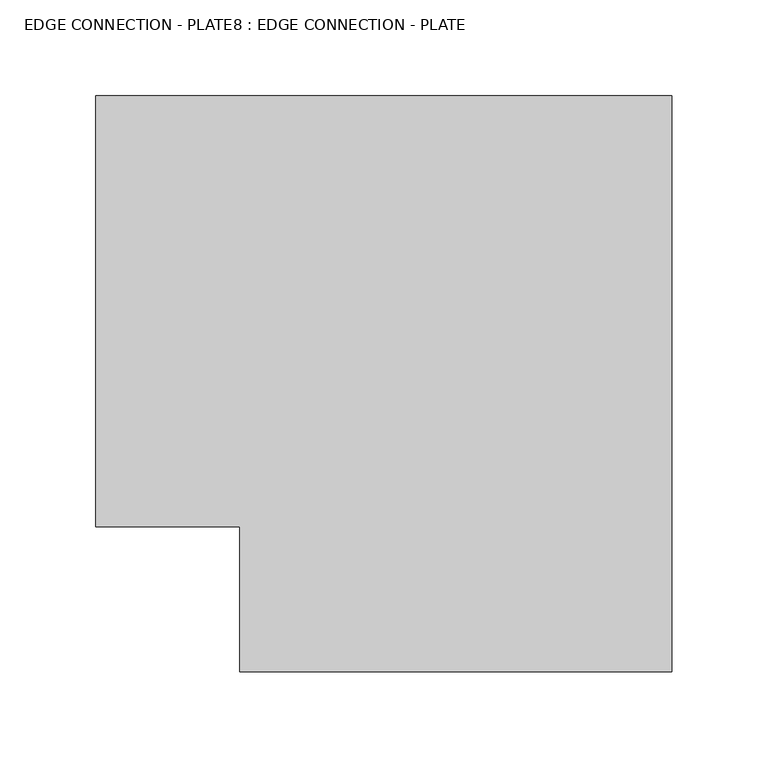
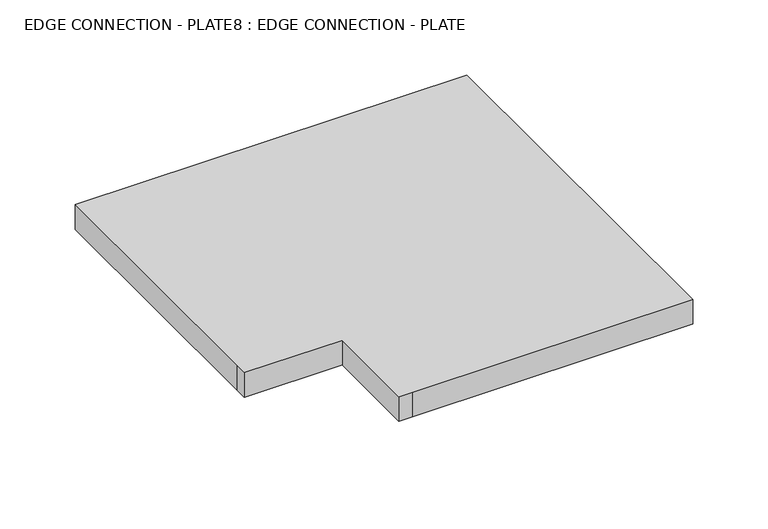
"""IFC4 building model written with IfcOpenShell, lengths in millimetres: fastener geometry, EDGE CONNECTION - PLATE8 : EDGE CONNECTION - PLATE."""

from ifc_helpers import new_model, si_unit, frame, origin, place, context, project, spatial, polyline, outline, extrude, source, transform, mapped, element, save


def edge_connection_plate8_edge_connection_plate_441fdba4(model_context):
    return source(origin(), model_context, "Body", "SweptSolid", [
        extrude(outline(polyline([(29700.0, 25499.5208589), (30000.0, 25499.5208589), (30000.0, 25199.5208589), (29784.862, 25199.5208589), (29774.862, 25199.5208589), (29774.862, 25275.0508589), (29700.0, 25275.0508589), (29700.0, 25285.0508589), (29700.0, 25499.5208589)])), frame((0.0, 0.0, 200.0), z_axis=(0.0, 0.0, 1.0), x_axis=(1.0, 0.0, 0.0)), (0.0, 0.0, 1.0), 20.0),
    ])


if __name__ == "__main__":
    model = new_model("IFC4")
    model_context = context("Model", 3, world=origin())
    ifc_project = project(units=[si_unit("LENGTHUNIT", "METRE", prefix="MILLI")], contexts=[model_context])
    site = spatial("IfcSite", under=ifc_project)
    building = spatial("IfcBuilding", under=site)
    placement = place(None, origin())
    edge_connection_plate8_edge_connection_plate_shape = edge_connection_plate8_edge_connection_plate_441fdba4(model_context)
    element("IfcFastener", 1, ObjectType="EDGE CONNECTION - PLATE8 : EDGE CONNECTION - PLATE", at=placement, inside=building, context=model_context, shape_type="MappedRepresentation", body=[
        mapped(edge_connection_plate8_edge_connection_plate_shape, transform((0.0, 0.0, 0.0), x_axis=(1.0, 0.0, 0.0), y_axis=(0.0, 1.0, 0.0), z_axis=(0.0, 0.0, 1.0))),
    ])
    save(model, "model.ifc")
